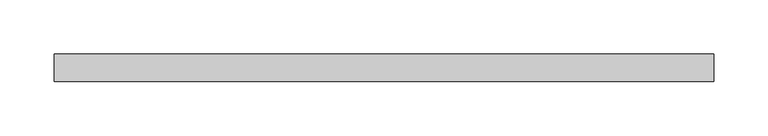
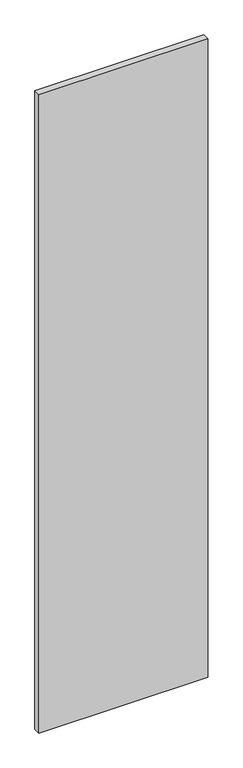
"""IFC4 building model written with IfcOpenShell, lengths in millimetres: proxy geometry, Vertical furring:Vertical furring:300288:Vertical furring:300288 : Vertical furring:Vertical furring:300288:300029:Vertical furring:300288:Vertical furring:300288 : Vertical furring:Vertical furring:300288:300029 : Vertical furring:Vertical furring:300288:Vertical furring:300288 : Vertical furring:Vertical furring:300288:300029:2 : Vertical furring:Vertical furring:300288:Vertical furring:300288 : Vertical furring:Vertical furring:300288:300029:Vertical furring:300288:Vertical furring:300288 : Vertical furring:Vertical furring:300288:300029 : Vertical furring:Vertical furring:300288:Vertical furring:300288 : Vertical furring:Vertical furring:300288:300029:300008."""

from ifc_helpers import new_model, si_unit, frame, origin, place, context, project, spatial, polyline, outline, extrude, source, transform, mapped, element, save


def generic_models_c4659f68(model_context):
    return source(origin(), model_context, "Body", "SweptSolid", [
        extrude(outline(polyline([(570455.7004145, -579025.9800746), (571065.3004145, -579025.9800746), (571065.3004145, -579051.3800746), (570455.7004145, -579051.3800746), (570455.7004145, -579025.9800746)])), frame((0.0, 0.0, 12.7), z_axis=(0.0, 0.0, 1.0), x_axis=(1.0, 0.0, 0.0)), (0.0, 0.0, 1.0), 2438.4),
    ])


if __name__ == "__main__":
    model = new_model("IFC4")
    model_context = context("Model", 3, world=origin())
    ifc_project = project(units=[si_unit("LENGTHUNIT", "METRE", prefix="MILLI")], contexts=[model_context])
    site = spatial("IfcSite", under=ifc_project)
    building = spatial("IfcBuilding", under=site)
    placement = place(None, origin())
    generic_models_shape = generic_models_c4659f68(model_context)
    element("IfcBuildingElementProxy", 1, Name="Vertical furring:Vertical furring:300288:Vertical furring:300288 : Vertical furring:Vertical furring:300288:300029:Vertical furring:300288:Vertical furring:300288 : Vertical furring:Vertical furring:300288:300029 : Vertical furring:Vertical furring:300288:Vertical furring:300288 : Vertical furring:Vertical furring:300288:300029:2 : Vertical furring:Vertical furring:300288:Vertical furring:300288 : Vertical furring:Vertical furring:300288:300029:Vertical furring:300288:Vertical furring:300288 : Vertical furring:Vertical furring:300288:300029 : Vertical furring:Vertical furring:300288:Vertical furring:300288 : Vertical furring:Vertical furring:300288:300029:300008", ObjectType="Vertical furring:Vertical furring:300288:Vertical furring:300288 : Vertical furring:Vertical furring:300288:300029:Vertical furring:300288:Vertical furring:300288 : Vertical furring:Vertical furring:300288:300029 : Vertical furring:Vertical furring:300288:Vertical furring:300288 : Vertical furring:Vertical furring:300288:300029:2 : Vertical furring:Vertical furring:300288:Vertical furring:300288 : Vertical furring:Vertical furring:300288:300029:Vertical furring:300288:Vertical furring:300288 : Vertical furring:Vertical furring:300288:300029 : Vertical furring:Vertical furring:300288:Vertical furring:300288 : Vertical furring:Vertical furring:300288:300029:300008", at=placement, inside=building, context=model_context, shape_type="MappedRepresentation", body=[
        mapped(generic_models_shape, transform((0.0, 0.0, 0.0), x_axis=(1.0, 0.0, 0.0), y_axis=(0.0, 1.0, 0.0), z_axis=(0.0, 0.0, 1.0))),
    ])
    save(model, "model.ifc")

# Revit data of these elements
# Type "Vertical furring:Vertical furring:300288:Vertical furring:300288 : Vertical furring:Vertical furring:300288:300029:Vertical furring:300288:Vertical furring:300288 : Vertical furring:Vertical furring:300288:300029 : Vertical furring:Vertical furring:300288:Vertical furring:300288 : Vertical furring:Vertical furring:300288:300029:2 : Vertical furring:Vertical furring:300288:Vertical furring:300288 : Vertical furring:Vertical furring:300288:300029:Vertical furring:300288:Vertical furring:300288 : Vertical furring:Vertical furring:300288:300029 : Vertical furring:Vertical furring:300288:Vertical furring:300288 : Vertical furring:Vertical furring:300288:300029:300008"
#   NameOverride = "Vertical furring:Vertical furring:300288:Vertical furring:300288 : Vertical furring:Vertical furring:300288:300029:Vertical furring:300288:Vertical furring:300288 : Vertical furring:Vertical furring:300288:300029 : Vertical furring:Vertical furring:300288:Vertical furring:300288 : Vertical furring:Vertical furring:300288:300029:300008"
#   ObjectTypeOverride = "Vertical furring:300288:Vertical furring:300288 : Vertical furring:Vertical furring:300288:300029 : Vertical furring:Vertical furring:300288:Vertical furring:300288 : Vertical furring:Vertical furring:300288:300029"
#   Reference = "Vertical furring"
#   Tag = "300008"
# Element 1 (IfcBuildingElementProxy, "Vertical furring:Vertical furring:300288:Vertical furring:300288 : Vertical furring:Vertical furring:300288:300029:Vertical furring:300288:Vertical furring:300288 : Vertical furring:Vertical furring:300288:300029 : Vertical furring:Vertical furring:300288:Vertical furring:300288 : Vertical furring:Vertical furring:300288:300029:2 : Vertical furring:Vertical furring:300288:Vertical furring:300288 : Vertical furring:Vertical furring:300288:300029:Vertical furring:300288:Vertical furring:300288 : Vertical furring:Vertical furring:300288:300029 : Vertical furring:Vertical furring:300288:Vertical furring:300288 : Vertical furring:Vertical furring:300288:300029:300008")
#   Materials on its faces: "1\" MINERAL WOOL BOARD INSULATION - BLACK MAT FACER"
# Materials
#   "1\" MINERAL WOOL BOARD INSULATION - BLACK MAT FACER": class "Unassigned", colour RGB 205 188 106, transparency 0, Cost = 0
